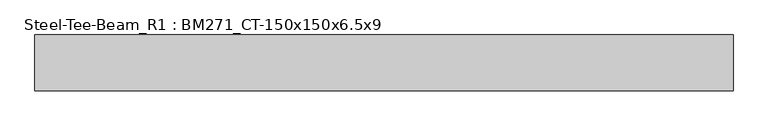
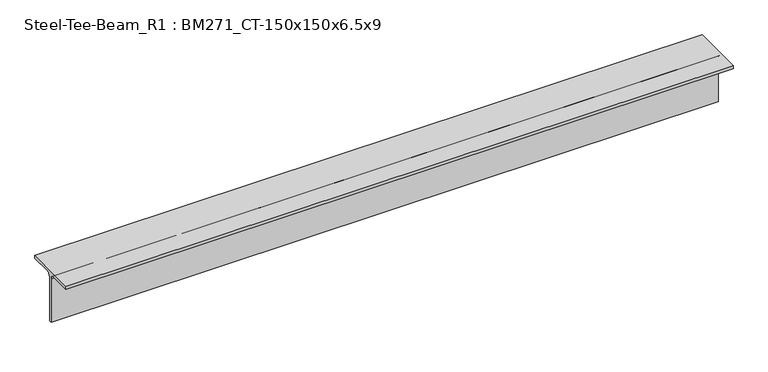
"""IFC4 building model written with IfcOpenShell, lengths in millimetres: member geometry, Steel-Tee-Beam_R1 : BM271_CT-150x150x6.5x9."""

from ifc_helpers import new_model, si_unit, point, frame, frame_2d, origin, place, context, project, spatial, polyline, circle_curve, trimmed, segment, composite_curve, outline, extrude, source, transform, mapped, element, save


def steel_tee_beam_r1_bm271_ct_150x150x6_5x9_d662a808(model_context):
    return source(origin(), model_context, "Body", "SweptSolid", [
        extrude(outline(composite_curve([segment(polyline([(-75.0, 75.0), (75.0, 75.0), (75.0, 66.0), (16.25, 66.0)]), True, "CONTINUOUS"), segment(trimmed(circle_curve(frame_2d((16.25, 53.0)), 13.0), [point((16.25, 66.0))], [point((3.25, 53.0))], True, "CARTESIAN"), True, "CONTINUOUS"), segment(polyline([(3.25, 53.0), (3.25, -75.0), (-3.25, -75.0), (-3.25, 53.0)]), True, "CONTINUOUS"), segment(trimmed(circle_curve(frame_2d((-16.25, 53.0)), 13.0), [point((-3.25, 53.0))], [point((-16.25, 66.0))], True, "CARTESIAN"), True, "CONTINUOUS"), segment(polyline([(-16.25, 66.0), (-75.0, 66.0), (-75.0, 75.0)]), True, "CONTINUOUS")], self_intersect=False)), frame((-1113.6541462, 0.0, 0.0), z_axis=(1.0, 0.0, 0.0), x_axis=(0.0, 1.0, 0.0)), (0.0, 0.0, 1.0), 1868.963443),
    ])


if __name__ == "__main__":
    model = new_model("IFC4")
    model_context = context("Model", 3, world=origin())
    ifc_project = project(units=[si_unit("LENGTHUNIT", "METRE", prefix="MILLI")], contexts=[model_context])
    site = spatial("IfcSite", under=ifc_project)
    building = spatial("IfcBuilding", under=site)
    placement = place(None, origin())
    steel_tee_beam_r1_bm271_ct_150x150x6_5x9_shape = steel_tee_beam_r1_bm271_ct_150x150x6_5x9_d662a808(model_context)
    element("IfcMember", 1, ObjectType="Steel-Tee-Beam_R1 : BM271_CT-150x150x6.5x9", at=placement, inside=building, context=model_context, shape_type="MappedRepresentation", body=[
        mapped(steel_tee_beam_r1_bm271_ct_150x150x6_5x9_shape, transform((0.0, 0.0, 0.0), x_axis=(1.0, 0.0, 0.0), y_axis=(0.0, 1.0, 0.0), z_axis=(0.0, 0.0, 1.0))),
    ])
    save(model, "model.ifc")

# Revit data of these elements
# Type "Steel-Tee-Beam_R1 : BM271_CT-150x150x6.5x9"
#   Keynote = "CT-150x150x6.5x9"
#   Surface Area = 0.588841 m²/m
#   Section Area = 23.3904 cm²
#   Mass per Unit Length = 18.3614 kg/m
#   Length [instance default] = 1.5240 m
#   bf = 0.1500 m
#   d = 0.1500 m
#   k = 0.0220 m
#   r = 0.0130 m
#   tf = 0.0090 m
#   tw = 0.0065 m
#   hec_material4 [instance default] = none
#   hec_material3 [instance default] = none
#   hec_material2 [instance default] = none
#   hec_material1 [instance default] = none
#   Structural Material [instance default] = Steel, 45-345
#   Assembly Code = ""
# Element 1 (IfcMember, "Steel-Tee-Beam_R1 : BM271_CT-150x150x6.5x9")
#   Structural Material = none
# Materials
#   "Steel, 45-345": class "Metal", colour RGB 189 187 185, transparency 0, Description = "Steel 345 MPa", Cost = 0
